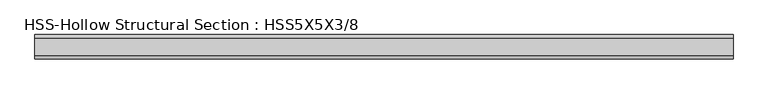
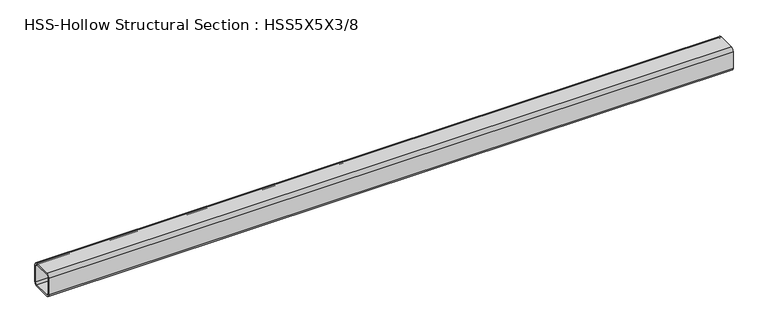
"""IFC4 building model written with IfcOpenShell, lengths in millimetres: beam geometry, HSS-Hollow Structural Section : HSS5X5X3/8."""

from ifc_helpers import new_model, si_unit, point, frame, frame_2d, origin, place, context, project, spatial, polyline, circle_curve, trimmed, segment, composite_curve, outline, extrude, source, transform, mapped, element, save


def hss_hollow_structural_section_hss5x5x3_8_57e97866(model_context):
    return source(origin(), model_context, "Body", "SweptSolid", [
        extrude(outline(composite_curve([segment(polyline([(63.5, 45.7708), (63.5, -45.7708)]), True, "CONTINUOUS"), segment(trimmed(circle_curve(frame_2d((45.7708, -45.7708)), 17.7292), [point((63.5, -45.7708))], [point((45.7708, -63.5))], False, "CARTESIAN"), True, "CONTINUOUS"), segment(polyline([(45.7708, -63.5), (-45.7708, -63.5)]), True, "CONTINUOUS"), segment(trimmed(circle_curve(frame_2d((-45.7708, -45.7708)), 17.7292), [point((-45.7708, -63.5))], [point((-63.5, -45.7708))], False, "CARTESIAN"), True, "CONTINUOUS"), segment(polyline([(-63.5, -45.7708), (-63.5, 45.7708)]), True, "CONTINUOUS"), segment(trimmed(circle_curve(frame_2d((-45.7708, 45.7708)), 17.7292), [point((-63.5, 45.7708))], [point((-45.7708, 63.5))], False, "CARTESIAN"), True, "CONTINUOUS"), segment(polyline([(-45.7708, 63.5), (45.7708, 63.5)]), True, "CONTINUOUS"), segment(trimmed(circle_curve(frame_2d((45.7708, 45.7708)), 17.7292), [point((45.7708, 63.5))], [point((63.5, 45.7708))], False, "CARTESIAN"), True, "CONTINUOUS")], self_intersect=False), holes=[composite_curve([segment(trimmed(circle_curve(frame_2d((-45.7708, 45.7708)), 8.8646), [point((-45.7708, 54.6354))], [point((-54.6354, 45.7708))], True, "CARTESIAN"), True, "CONTINUOUS"), segment(polyline([(-54.6354, 45.7708), (-54.6354, -45.7708)]), True, "CONTINUOUS"), segment(trimmed(circle_curve(frame_2d((-45.7708, -45.7708)), 8.8646), [point((-54.6354, -45.7708))], [point((-45.7708, -54.6354))], True, "CARTESIAN"), True, "CONTINUOUS"), segment(polyline([(-45.7708, -54.6354), (45.7708, -54.6354)]), True, "CONTINUOUS"), segment(trimmed(circle_curve(frame_2d((45.7708, -45.7708)), 8.8646), [point((45.7708, -54.6354))], [point((54.6354, -45.7708))], True, "CARTESIAN"), True, "CONTINUOUS"), segment(polyline([(54.6354, -45.7708), (54.6354, 45.7708)]), True, "CONTINUOUS"), segment(trimmed(circle_curve(frame_2d((45.7708, 45.7708)), 8.8646), [point((54.6354, 45.7708))], [point((45.7708, 54.6354))], True, "CARTESIAN"), True, "CONTINUOUS"), segment(polyline([(45.7708, 54.6354), (-45.7708, 54.6354)]), True, "CONTINUOUS")], self_intersect=False)]), frame((-1812.925, 0.0, 0.0), z_axis=(1.0, 0.0, 0.0), x_axis=(0.0, 1.0, 0.0)), (0.0, 0.0, 1.0), 3625.85),
    ])


if __name__ == "__main__":
    model = new_model("IFC4")
    model_context = context("Model", 3, world=origin())
    ifc_project = project(units=[si_unit("LENGTHUNIT", "METRE", prefix="MILLI")], contexts=[model_context])
    site = spatial("IfcSite", under=ifc_project)
    building = spatial("IfcBuilding", under=site)
    placement = place(None, origin())
    hss_hollow_structural_section_hss5x5x3_8_shape = hss_hollow_structural_section_hss5x5x3_8_57e97866(model_context)
    element("IfcBeam", 1, ObjectType="HSS-Hollow Structural Section : HSS5X5X3/8", at=placement, inside=building, context=model_context, shape_type="MappedRepresentation", body=[
        mapped(hss_hollow_structural_section_hss5x5x3_8_shape, transform((0.0, 0.0, 0.0), x_axis=(1.0, 0.0, 0.0), y_axis=(0.0, 1.0, 0.0), z_axis=(0.0, 0.0, 1.0))),
    ])
    save(model, "model.ifc")

# Revit data of these elements
# Type "HSS-Hollow Structural Section : HSS5X5X3/8"
#   Assembly Code = "B10"
#   Shape = "Square"
#   W = 22.3
#   Ht = 0' - 5"
#   Length [instance default] = 5' - 0"
#   b = 0' - 5"
#   kr = 0' - 0.698"
#   t = 0' - 0.349"
#   A = 0.0429167 SF
#   Structural Material [instance default] = Steel ASTM A500, Grade B, Rectangular and Square
# Element 1 (IfcBeam, "HSS-Hollow Structural Section : HSS5X5X3/8")
#   Materials on its faces: "Steel ASTM A500, Grade B, Rectangular and Square"
# Materials
#   "Steel ASTM A500, Grade B, Rectangular and Square": class "Metal", colour RGB 199 199 199, transparency 0, Description = "Carbon steel", Cost = 0
